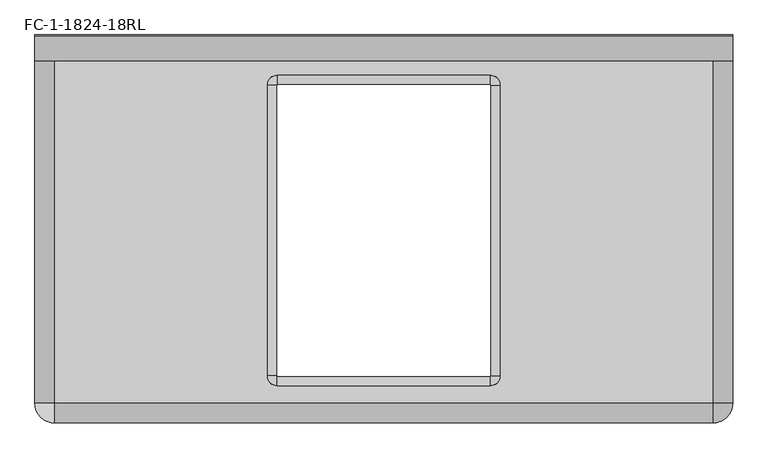
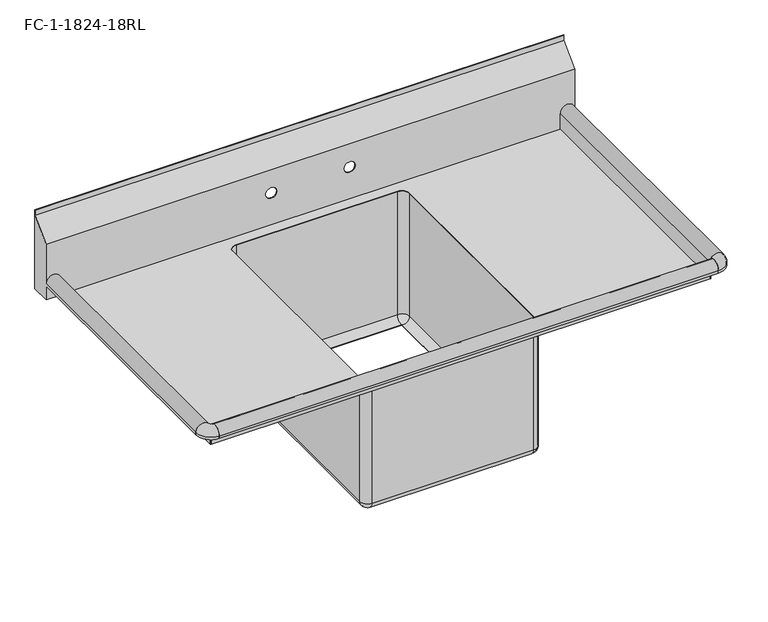
"""IFC4 building model written with IfcOpenShell, lengths in millimetres: proxy geometry, qf_advance_fc-1$2014$FC-1-1824-18RL : FC-1-1824-18RL."""

from ifc_helpers import new_model, si_unit, point, frame, frame_2d, origin, place, context, project, spatial, polyline, circle_curve, ellipse_curve, trimmed, segment, composite_curve, outline, extrude, source, transform, mapped, element, save
from ifc_brep_helpers import plane_surface, cylinder_surface, revolved_surface, advanced_brep


def fc_1_1824_18rl_eb121c77(model_context):
    return source(origin(), model_context, "Body", "SolidModel", [
        advanced_brep(
        [(915.9680523, -98.425, 539.7540518), (895.35, -77.8069477, 539.7540518), (895.35, -77.8069477, 876.3), (915.9680523, -98.425, 876.3), (896.9063565, -98.425, 520.692356), (895.35, -96.8686435, 520.692356), (896.9063565, -98.425, 522.2798689), (895.35, -96.8686435, 522.2798689), (914.3805538, -98.425, 539.7540662), (895.35, -79.3944462, 539.7540662), (914.3805538, -98.425, 876.3), (895.35, -79.3944462, 876.3), (915.9680523, -669.925, 876.3), (915.9680523, -669.925, 539.7540518), (896.9063565, -669.925, 520.692356), (896.9063565, -669.925, 522.2798689), (914.3805538, -669.925, 539.7540662), (914.3805538, -669.925, 876.3), (895.35, -690.5430523, 539.7540518), (895.35, -690.5430523, 876.3), (895.35, -671.4813565, 520.692356), (895.35, -671.4813565, 522.2798689), (895.35, -688.9555538, 539.7540662), (895.35, -688.9555538, 876.3), (476.25, -690.5430523, 876.3), (476.25, -690.5430523, 539.7540518), (476.25, -671.4813565, 520.692356), (476.25, -671.4813565, 522.2798689), (476.25, -688.9555538, 539.7540662), (476.25, -688.9555538, 876.3), (455.6319477, -669.925, 539.7540518), (455.6319477, -669.925, 876.3), (474.6936435, -669.925, 520.692356), (474.6936435, -669.925, 522.2798689), (457.2194462, -669.925, 539.7540662), (457.2194462, -669.925, 876.3), (455.6319477, -98.425, 876.3), (455.6319477, -98.425, 539.7540518), (474.6936435, -98.425, 520.692356), (474.6936435, -98.425, 522.2798689), (457.2194462, -98.425, 539.7540662), (457.2194462, -98.425, 876.3), (476.25, -77.8069477, 539.7540518), (476.25, -77.8069477, 876.3), (476.25, -96.8686435, 520.692356), (476.25, -96.8686435, 522.2798689), (476.25, -79.3944462, 539.7540662), (476.25, -79.3944462, 876.3)],
        [
            (0, 1, circle_curve(frame((895.35, -98.425, 539.7540518), z_axis=(0.0, 0.0, 1.0), x_axis=(0.0, 1.0, 0.0)), 20.6180523)),
            (1, 2),
            (2, 3, circle_curve(frame((895.35, -98.425, 876.3), z_axis=(0.0, 0.0, -1.0), x_axis=(0.0, 1.0, 0.0)), 20.6180523)),
            (3, 0),
            (4, 5, circle_curve(frame((895.35, -98.425, 520.692356), z_axis=(0.0, 0.0, 1.0), x_axis=(0.0, 1.0, 0.0)), 1.5563565)),
            (5, 1, circle_curve(frame((895.35, -96.8686435, 539.7540518), z_axis=(1.0, 0.0, 0.0), x_axis=(0.0, 1.0, 0.0)), 19.0616958)),
            (0, 4, circle_curve(frame((896.9063565, -98.425, 539.7540518), z_axis=(0.0, 1.0, 0.0), x_axis=(1.0, 0.0, 0.0)), 19.0616958)),
            (6, 7, circle_curve(frame((895.35, -98.425, 522.2798689), z_axis=(0.0, 0.0, 1.0), x_axis=(0.0, 1.0, 0.0)), 1.5563565)),
            (7, 5),
            (4, 6),
            (8, 9, circle_curve(frame((895.35, -98.425, 539.7540662), z_axis=(0.0, 0.0, 1.0), x_axis=(0.0, 1.0, 0.0)), 19.0305538)),
            (9, 7, circle_curve(frame((895.35, -96.8686435, 539.7540662), z_axis=(-1.0, 0.0, 0.0), x_axis=(0.0, 1.0, 0.0)), 17.4741973)),
            (6, 8, circle_curve(frame((896.9063565, -98.425, 539.7540662), z_axis=(0.0, -1.0, 0.0), x_axis=(1.0, 0.0, 0.0)), 17.4741973)),
            (10, 11, circle_curve(frame((895.35, -98.425, 876.3), z_axis=(0.0, 0.0, 1.0), x_axis=(0.0, 1.0, 0.0)), 19.0305538)),
            (11, 9),
            (8, 10),
            (3, 12),
            (12, 13),
            (13, 0),
            (13, 14, circle_curve(frame((896.9063565, -669.925, 539.7540518), z_axis=(0.0, 1.0, 0.0), x_axis=(1.0, 0.0, 0.0)), 19.0616958)),
            (14, 4),
            (14, 15),
            (15, 6),
            (15, 16, circle_curve(frame((896.9063565, -669.925, 539.7540662), z_axis=(0.0, -1.0, 0.0), x_axis=(1.0, 0.0, 0.0)), 17.4741973)),
            (16, 8),
            (16, 17),
            (17, 10),
            (18, 13, circle_curve(frame((895.35, -669.925, 539.7540518), z_axis=(0.0, 0.0, 1.0), x_axis=(1.0, 0.0, 0.0)), 20.6180523)),
            (12, 19, circle_curve(frame((895.35, -669.925, 876.3), z_axis=(0.0, 0.0, -1.0), x_axis=(1.0, 0.0, 0.0)), 20.6180523)),
            (19, 18),
            (20, 14, circle_curve(frame((895.35, -669.925, 520.692356), z_axis=(0.0, 0.0, 1.0), x_axis=(1.0, 0.0, 0.0)), 1.5563565)),
            (18, 20, circle_curve(frame((895.35, -671.4813565, 539.7540518), z_axis=(1.0, 0.0, 0.0), x_axis=(0.0, -1.0, 0.0)), 19.0616958)),
            (21, 15, circle_curve(frame((895.35, -669.925, 522.2798689), z_axis=(0.0, 0.0, 1.0), x_axis=(1.0, 0.0, 0.0)), 1.5563565)),
            (20, 21),
            (22, 16, circle_curve(frame((895.35, -669.925, 539.7540662), z_axis=(0.0, 0.0, 1.0), x_axis=(1.0, 0.0, 0.0)), 19.0305538)),
            (21, 22, circle_curve(frame((895.35, -671.4813565, 539.7540662), z_axis=(-1.0, 0.0, 0.0), x_axis=(0.0, -1.0, 0.0)), 17.4741973)),
            (23, 17, circle_curve(frame((895.35, -669.925, 876.3), z_axis=(0.0, 0.0, 1.0), x_axis=(1.0, 0.0, 0.0)), 19.0305538)),
            (22, 23),
            (19, 24),
            (24, 25),
            (25, 18),
            (25, 26, circle_curve(frame((476.25, -671.4813565, 539.7540518), z_axis=(1.0, 0.0, 0.0), x_axis=(0.0, -1.0, 0.0)), 19.0616958)),
            (26, 20),
            (26, 27),
            (27, 21),
            (27, 28, circle_curve(frame((476.25, -671.4813565, 539.7540662), z_axis=(-1.0, 0.0, 0.0), x_axis=(0.0, -1.0, 0.0)), 17.4741973)),
            (28, 22),
            (28, 29),
            (29, 23),
            (30, 25, circle_curve(frame((476.25, -669.925, 539.7540518), z_axis=(0.0, 0.0, 1.0), x_axis=(0.0, -1.0, 0.0)), 20.6180523)),
            (24, 31, circle_curve(frame((476.25, -669.925, 876.3), z_axis=(0.0, 0.0, -1.0), x_axis=(0.0, -1.0, 0.0)), 20.6180523)),
            (31, 30),
            (32, 26, circle_curve(frame((476.25, -669.925, 520.692356), z_axis=(0.0, 0.0, 1.0), x_axis=(0.0, -1.0, 0.0)), 1.5563565)),
            (30, 32, circle_curve(frame((474.6936435, -669.925, 539.7540518), z_axis=(0.0, -1.0, 0.0), x_axis=(-1.0, 0.0, 0.0)), 19.0616958)),
            (33, 27, circle_curve(frame((476.25, -669.925, 522.2798689), z_axis=(0.0, 0.0, 1.0), x_axis=(0.0, -1.0, 0.0)), 1.5563565)),
            (32, 33),
            (34, 28, circle_curve(frame((476.25, -669.925, 539.7540662), z_axis=(0.0, 0.0, 1.0), x_axis=(0.0, -1.0, 0.0)), 19.0305538)),
            (33, 34, circle_curve(frame((474.6936435, -669.925, 539.7540662), z_axis=(0.0, 1.0, 0.0), x_axis=(-1.0, 0.0, 0.0)), 17.4741973)),
            (35, 29, circle_curve(frame((476.25, -669.925, 876.3), z_axis=(0.0, 0.0, 1.0), x_axis=(0.0, -1.0, 0.0)), 19.0305538)),
            (34, 35),
            (31, 36),
            (36, 37),
            (37, 30),
            (37, 38, circle_curve(frame((474.6936435, -98.425, 539.7540518), z_axis=(0.0, -1.0, 0.0), x_axis=(-1.0, 0.0, 0.0)), 19.0616958)),
            (38, 32),
            (38, 39),
            (39, 33),
            (39, 40, circle_curve(frame((474.6936435, -98.425, 539.7540662), z_axis=(0.0, 1.0, 0.0), x_axis=(-1.0, 0.0, 0.0)), 17.4741973)),
            (40, 34),
            (40, 41),
            (41, 35),
            (42, 37, circle_curve(frame((476.25, -98.425, 539.7540518), z_axis=(0.0, 0.0, 1.0), x_axis=(-1.0, 0.0, 0.0)), 20.6180523)),
            (36, 43, circle_curve(frame((476.25, -98.425, 876.3), z_axis=(0.0, 0.0, -1.0), x_axis=(-1.0, 0.0, 0.0)), 20.6180523)),
            (43, 42),
            (44, 38, circle_curve(frame((476.25, -98.425, 520.692356), z_axis=(0.0, 0.0, 1.0), x_axis=(-1.0, 0.0, 0.0)), 1.5563565)),
            (42, 44, circle_curve(frame((476.25, -96.8686435, 539.7540518), z_axis=(-1.0, 0.0, 0.0), x_axis=(0.0, 1.0, 0.0)), 19.0616958)),
            (45, 39, circle_curve(frame((476.25, -98.425, 522.2798689), z_axis=(0.0, 0.0, 1.0), x_axis=(-1.0, 0.0, 0.0)), 1.5563565)),
            (44, 45),
            (46, 40, circle_curve(frame((476.25, -98.425, 539.7540662), z_axis=(0.0, 0.0, 1.0), x_axis=(-1.0, 0.0, 0.0)), 19.0305538)),
            (45, 46, circle_curve(frame((476.25, -96.8686435, 539.7540662), z_axis=(1.0, 0.0, 0.0), x_axis=(0.0, 1.0, 0.0)), 17.4741973)),
            (47, 41, circle_curve(frame((476.25, -98.425, 876.3), z_axis=(0.0, 0.0, 1.0), x_axis=(-1.0, 0.0, 0.0)), 19.0305538)),
            (46, 47),
            (43, 2),
            (1, 42),
            (5, 44),
            (7, 45),
            (9, 46),
            (11, 47),
        ],
        [
            cylinder_surface(frame((895.35, -98.425, 0.0), z_axis=(0.0, 0.0, -1.0), x_axis=(0.0, 1.0, 0.0)), 20.6180523),
            revolved_surface(trimmed(ellipse_curve(frame((895.35, -96.8686435, 539.7540518), z_axis=(-1.0, 0.0, 0.0), x_axis=(0.0, 1.0, 0.0)), 19.0616958, 19.0616958), [point((895.35, -77.8069477, 539.7540518))], [point((895.35, -96.8686435, 520.692356))], True, "CARTESIAN"), (895.35, -98.425, 0.0), (0.0, 0.0, -1.0)),
            revolved_surface(polyline([(895.35, -96.86864349999999, 520.692356), (895.35, -96.86864349999999, 522.2798689)]), (895.35, -98.425, 0.0), (0.0, 0.0, -1.0)),
            revolved_surface(trimmed(ellipse_curve(frame((895.35, -96.8686435, 539.7540662), z_axis=(1.0, 0.0, 0.0), x_axis=(0.0, 1.0, 0.0)), 17.4741973, 17.4741973), [point((895.35, -96.8686435, 522.2798689))], [point((895.35, -79.3944462, 539.7540662))], True, "CARTESIAN"), (895.35, -98.425, 0.0), (0.0, 0.0, -1.0)),
            revolved_surface(polyline([(895.35, -79.3944462, 539.7540662), (895.35, -79.3944462, 876.3)]), (895.35, -98.425, 0.0), (0.0, 0.0, -1.0)),
            plane_surface(frame((915.9680523, -98.425, 876.3), z_axis=(1.0, 0.0, 0.0), x_axis=(0.0, -1.0, 0.0))),
            cylinder_surface(frame((896.9063565, -98.425, 539.7540518), z_axis=(0.0, 1.0, 0.0), x_axis=(1.0, 0.0, 0.0)), 19.0616958),
            plane_surface(frame((896.9063565, -98.425, 520.692356), z_axis=(-1.0, 0.0, 0.0), x_axis=(0.0, -1.0, 0.0))),
            revolved_surface(polyline([(914.3805538, -669.925, 539.7540662), (914.3805538, -98.425, 539.7540662)]), (896.9063565, -98.425, 539.7540662), (0.0, -1.0, 0.0)),
            plane_surface(frame((914.3805538, -98.425, 539.7540662), z_axis=(-1.0, 0.0, 0.0), x_axis=(0.0, -1.0, 0.0))),
            cylinder_surface(frame((895.35, -669.925, 0.0), z_axis=(0.0, 0.0, -1.0), x_axis=(1.0, 0.0, 0.0)), 20.6180523),
            revolved_surface(trimmed(ellipse_curve(frame((896.9063565, -669.925, 539.7540518), z_axis=(0.0, 1.0, 0.0), x_axis=(1.0, 0.0, 0.0)), 19.0616958, 19.0616958), [point((915.9680523, -669.925, 539.7540518))], [point((896.9063565, -669.925, 520.692356))], True, "CARTESIAN"), (895.35, -669.925, 0.0), (0.0, 0.0, -1.0)),
            revolved_surface(polyline([(896.9063565, -669.925, 520.692356), (896.9063565, -669.925, 522.2798689)]), (895.35, -669.925, 0.0), (0.0, 0.0, -1.0)),
            revolved_surface(trimmed(ellipse_curve(frame((896.9063565, -669.925, 539.7540662), z_axis=(0.0, -1.0, 0.0), x_axis=(1.0, 0.0, 0.0)), 17.4741973, 17.4741973), [point((896.9063565, -669.925, 522.2798689))], [point((914.3805538, -669.925, 539.7540662))], True, "CARTESIAN"), (895.35, -669.925, 0.0), (0.0, 0.0, -1.0)),
            revolved_surface(polyline([(914.3805538, -669.925, 539.7540662), (914.3805538, -669.925, 876.3)]), (895.35, -669.925, 0.0), (0.0, 0.0, -1.0)),
            plane_surface(frame((895.35, -690.5430523, 876.3), z_axis=(0.0, -1.0, 0.0), x_axis=(-1.0, 0.0, 0.0))),
            cylinder_surface(frame((895.35, -671.4813565, 539.7540518), z_axis=(1.0, 0.0, 0.0), x_axis=(0.0, -1.0, 0.0)), 19.0616958),
            plane_surface(frame((895.35, -671.4813565, 520.692356), z_axis=(0.0, 1.0, 0.0), x_axis=(-1.0, 0.0, 0.0))),
            revolved_surface(polyline([(476.25, -688.9555538, 539.7540662), (895.35, -688.9555538, 539.7540662)]), (895.35, -671.4813565, 539.7540662), (-1.0, 0.0, 0.0)),
            plane_surface(frame((895.35, -688.9555538, 539.7540662), z_axis=(0.0, 1.0, 0.0), x_axis=(-1.0, 0.0, 0.0))),
            cylinder_surface(frame((476.25, -669.925, 0.0), z_axis=(0.0, 0.0, -1.0), x_axis=(0.0, -1.0, 0.0)), 20.6180523),
            revolved_surface(trimmed(ellipse_curve(frame((476.25, -671.4813565, 539.7540518), z_axis=(1.0, 0.0, 0.0), x_axis=(0.0, -1.0, 0.0)), 19.0616958, 19.0616958), [point((476.25, -690.5430523, 539.7540518))], [point((476.25, -671.4813565, 520.692356))], True, "CARTESIAN"), (476.25, -669.925, 0.0), (0.0, 0.0, -1.0)),
            revolved_surface(polyline([(476.25, -671.4813565, 520.692356), (476.25, -671.4813565, 522.2798689)]), (476.25, -669.925, 0.0), (0.0, 0.0, -1.0)),
            revolved_surface(trimmed(ellipse_curve(frame((476.25, -671.4813565, 539.7540662), z_axis=(-1.0, 0.0, 0.0), x_axis=(0.0, -1.0, 0.0)), 17.4741973, 17.4741973), [point((476.25, -671.4813565, 522.2798689))], [point((476.25, -688.9555538, 539.7540662))], True, "CARTESIAN"), (476.25, -669.925, 0.0), (0.0, 0.0, -1.0)),
            revolved_surface(polyline([(476.25, -688.9555538, 539.7540662), (476.25, -688.9555538, 876.3)]), (476.25, -669.925, 0.0), (0.0, 0.0, -1.0)),
            plane_surface(frame((455.6319477, -669.925, 876.3), z_axis=(-1.0, 0.0, 0.0), x_axis=(0.0, 1.0, 0.0))),
            cylinder_surface(frame((474.6936435, -669.925, 539.7540518), z_axis=(0.0, -1.0, 0.0), x_axis=(-1.0, 0.0, 0.0)), 19.0616958),
            plane_surface(frame((474.6936435, -669.925, 520.692356), z_axis=(1.0, 0.0, 0.0), x_axis=(0.0, 1.0, 0.0))),
            revolved_surface(polyline([(457.2194462, -98.42499999999995, 539.7540662), (457.2194462, -669.925, 539.7540662)]), (474.6936435, -669.925, 539.7540662), (0.0, 1.0, 0.0)),
            plane_surface(frame((457.2194462, -669.925, 539.7540662), z_axis=(1.0, 0.0, 0.0), x_axis=(0.0, 1.0, 0.0))),
            cylinder_surface(frame((476.25, -98.425, 0.0), z_axis=(0.0, 0.0, -1.0), x_axis=(-1.0, 0.0, 0.0)), 20.6180523),
            revolved_surface(trimmed(ellipse_curve(frame((474.6936435, -98.425, 539.7540518), z_axis=(0.0, -1.0, 0.0), x_axis=(-1.0, 0.0, 0.0)), 19.0616958, 19.0616958), [point((455.6319477, -98.425, 539.7540518))], [point((474.6936435, -98.425, 520.692356))], True, "CARTESIAN"), (476.25, -98.425, 0.0), (0.0, 0.0, -1.0)),
            revolved_surface(polyline([(474.6936435, -98.425, 520.692356), (474.6936435, -98.425, 522.2798689)]), (476.25, -98.425, 0.0), (0.0, 0.0, -1.0)),
            revolved_surface(trimmed(ellipse_curve(frame((474.6936435, -98.425, 539.7540662), z_axis=(0.0, 1.0, 0.0), x_axis=(-1.0, 0.0, 0.0)), 17.4741973, 17.4741973), [point((474.6936435, -98.425, 522.2798689))], [point((457.2194462, -98.425, 539.7540662))], True, "CARTESIAN"), (476.25, -98.425, 0.0), (0.0, 0.0, -1.0)),
            revolved_surface(polyline([(457.2194462, -98.425, 539.7540662), (457.2194462, -98.425, 876.3)]), (476.25, -98.425, 0.0), (0.0, 0.0, -1.0)),
            plane_surface(frame((476.25, -77.8069477, 876.3), z_axis=(0.0, 1.0, 0.0), x_axis=(1.0, 0.0, 0.0))),
            cylinder_surface(frame((476.25, -96.8686435, 539.7540518), z_axis=(-1.0, 0.0, 0.0), x_axis=(0.0, 1.0, 0.0)), 19.0616958),
            plane_surface(frame((476.25, -96.8686435, 520.692356), z_axis=(0.0, -1.0, 0.0), x_axis=(1.0, 0.0, 0.0))),
            revolved_surface(polyline([(895.35, -79.3944462, 539.7540662), (476.25, -79.3944462, 539.7540662)]), (476.25, -96.8686435, 539.7540662), (1.0, 0.0, 0.0)),
            plane_surface(frame((476.25, -79.3944462, 539.7540662), z_axis=(0.0, -1.0, 0.0), x_axis=(1.0, 0.0, 0.0))),
            plane_surface(frame((476.25, -79.3944462, 876.3), z_axis=(0.0, 0.0, 1.0), x_axis=(1.0, 0.0, 0.0))),
        ],
        [
            (0, [[1, 2, 3, 4]]),
            (1, [[5, 6, -1, 7]]),
            (2, [[8, 9, -5, 10]]),
            (3, [[11, 12, -8, 13]]),
            (4, [[14, 15, -11, 16]]),
            (5, [[-4, 17, 18, 19]]),
            (6, [[-7, -19, 20, 21]]),
            (7, [[-10, -21, 22, 23]]),
            (8, [[-13, -23, 24, 25]]),
            (9, [[-16, -25, 26, 27]]),
            (10, [[28, -18, 29, 30]]),
            (11, [[31, -20, -28, 32]]),
            (12, [[33, -22, -31, 34]]),
            (13, [[35, -24, -33, 36]]),
            (14, [[37, -26, -35, 38]]),
            (15, [[-30, 39, 40, 41]]),
            (16, [[-32, -41, 42, 43]]),
            (17, [[-34, -43, 44, 45]]),
            (18, [[-36, -45, 46, 47]]),
            (19, [[-38, -47, 48, 49]]),
            (20, [[50, -40, 51, 52]]),
            (21, [[53, -42, -50, 54]]),
            (22, [[55, -44, -53, 56]]),
            (23, [[57, -46, -55, 58]]),
            (24, [[59, -48, -57, 60]]),
            (25, [[-52, 61, 62, 63]]),
            (26, [[-54, -63, 64, 65]]),
            (27, [[-56, -65, 66, 67]]),
            (28, [[-58, -67, 68, 69]]),
            (29, [[-60, -69, 70, 71]]),
            (30, [[72, -62, 73, 74]]),
            (31, [[75, -64, -72, 76]]),
            (32, [[77, -66, -75, 78]]),
            (33, [[79, -68, -77, 80]]),
            (34, [[81, -70, -79, 82]]),
            (35, [[-74, 83, -2, 84]]),
            (36, [[-76, -84, -6, 85]]),
            (37, [[-78, -85, -9, 86]]),
            (38, [[-80, -86, -12, 87]]),
            (39, [[-82, -87, -15, 88]]),
            (40, [[-83, -73, -61, -51, -39, -29, -17, -3], [-71, -81, -88, -14, -27, -37, -49, -59]]),
        ],
    ),
        extrude(outline(polyline([(38.1, -723.9), (38.1, -50.8), (1333.5, -50.8), (1333.5, -723.9), (38.1, -723.9)]), holes=[composite_curve([segment(trimmed(circle_curve(frame_2d((895.35, -98.425)), 19.05), [point((914.4, -98.425))], [point((895.35, -79.375))], True, "CARTESIAN"), True, "CONTINUOUS"), segment(polyline([(895.35, -79.375), (476.25, -79.375)]), True, "CONTINUOUS"), segment(trimmed(circle_curve(frame_2d((476.25, -98.425)), 19.05), [point((476.25, -79.375))], [point((457.2, -98.425))], True, "CARTESIAN"), True, "CONTINUOUS"), segment(polyline([(457.2, -98.425), (457.2, -669.925)]), True, "CONTINUOUS"), segment(trimmed(circle_curve(frame_2d((476.25, -669.925)), 19.05), [point((457.2, -669.925))], [point((476.25, -688.975))], True, "CARTESIAN"), True, "CONTINUOUS"), segment(polyline([(476.25, -688.975), (895.35, -688.975)]), True, "CONTINUOUS"), segment(trimmed(circle_curve(frame_2d((895.35, -669.925)), 19.05), [point((895.35, -688.975))], [point((914.4, -669.925))], True, "CARTESIAN"), True, "CONTINUOUS"), segment(polyline([(914.4, -669.925), (914.4, -98.425)]), True, "CONTINUOUS")], self_intersect=False)]), frame((0.0, 0.0, 876.3), z_axis=(0.0, 0.0, 1.0), x_axis=(1.0, 0.0, 0.0)), (0.0, 0.0, 1.0), 1.5875),
        advanced_brep(
        [(38.1, -725.4875, 876.3), (38.1, -723.9, 876.3), (38.1, -723.9, 920.75), (38.1, -762.0, 920.75), (38.1, -762.0, 914.4), (38.1, -760.4125, 914.4), (38.1, -760.4125, 920.75), (38.1, -725.4875, 920.75), (36.5125, -723.9, 876.3), (36.5125, -723.9, 920.75), (1.5875, -723.9, 920.75), (1.5875, -723.9, 914.4), (0.0, -723.9, 914.4), (0.0, -723.9, 920.75)],
        [
            (0, 1),
            (1, 2),
            (2, 3, circle_curve(frame((38.1, -742.95, 920.75), z_axis=(1.0, 0.0, 0.0), x_axis=(0.0, -1.0, 0.0)), 19.05)),
            (3, 4),
            (4, 5),
            (5, 6),
            (6, 7, circle_curve(frame((38.1, -742.95, 920.75), z_axis=(-1.0, 0.0, 0.0), x_axis=(0.0, -1.0, 0.0)), 17.4625)),
            (7, 0),
            (8, 9),
            (9, 10, circle_curve(frame((19.05, -723.9, 920.75), z_axis=(0.0, -1.0, 0.0), x_axis=(-1.0, 0.0, 0.0)), 17.4625)),
            (10, 11),
            (11, 12),
            (12, 13),
            (13, 2, circle_curve(frame((19.05, -723.9, 920.75), z_axis=(0.0, 1.0, 0.0), x_axis=(-1.0, 0.0, 0.0)), 19.05)),
            (1, 8),
            (8, 0, circle_curve(frame((38.1, -723.9, 876.3), z_axis=(0.0, 0.0, 1.0), x_axis=(0.0, -1.0, 0.0)), 1.5875)),
            (7, 9, circle_curve(frame((38.1, -723.9, 920.75), z_axis=(0.0, 0.0, -1.0), x_axis=(0.0, -1.0, 0.0)), 1.5875)),
            (6, 10, circle_curve(frame((38.1, -723.9, 920.75), z_axis=(0.0, 0.0, -1.0), x_axis=(0.0, -1.0, 0.0)), 36.5125)),
            (5, 11, circle_curve(frame((38.1, -723.9, 914.4), z_axis=(0.0, 0.0, -1.0), x_axis=(0.0, -1.0, 0.0)), 36.5125)),
            (4, 12, circle_curve(frame((38.1, -723.9, 914.4), z_axis=(0.0, 0.0, -1.0), x_axis=(0.0, -1.0, 0.0)), 38.1)),
            (3, 13, circle_curve(frame((38.1, -723.9, 920.75), z_axis=(0.0, 0.0, -1.0), x_axis=(0.0, -1.0, 0.0)), 38.1)),
        ],
        [
            plane_surface(frame((38.1, -723.9, 876.3), z_axis=(1.0, 0.0, 0.0), x_axis=(0.0, -1.0, 0.0))),
            plane_surface(frame((38.1, -723.9, 876.3), z_axis=(0.0, 1.0, 0.0), x_axis=(-1.0, 0.0, 0.0))),
            cylinder_surface(frame((38.1, -723.9, 876.3), z_axis=(0.0, 0.0, -1.0), x_axis=(0.0, -1.0, 0.0)), 1.5875),
            revolved_surface(trimmed(ellipse_curve(frame((38.1, -742.95, 920.75), z_axis=(-1.0, 0.0, 0.0), x_axis=(0.0, -1.0, 0.0)), 17.4625, 17.4625), [point((38.1, -760.4125, 920.75))], [point((38.1, -725.4875, 920.75))], True, "CARTESIAN"), (38.1, -723.9, 876.3), (0.0, 0.0, -1.0)),
            revolved_surface(polyline([(38.1, -760.4125, 914.4), (38.1, -760.4125, 920.75)]), (38.1, -723.9, 876.3), (0.0, 0.0, -1.0)),
            plane_surface(frame((38.1, -723.9, 914.4), z_axis=(0.0, 0.0, -1.0), x_axis=(0.0, -1.0, 0.0))),
            cylinder_surface(frame((38.1, -723.9, 876.3), z_axis=(0.0, 0.0, -1.0), x_axis=(0.0, -1.0, 0.0)), 38.1),
            revolved_surface(trimmed(ellipse_curve(frame((38.1, -742.95, 920.75), z_axis=(1.0, 0.0, 0.0), x_axis=(0.0, -1.0, 0.0)), 19.05, 19.05), [point((38.1, -723.9, 920.75))], [point((38.1, -762.0, 920.75))], True, "CARTESIAN"), (38.1, -723.9, 876.3), (0.0, 0.0, -1.0)),
            plane_surface(frame((38.1, -723.9, 876.3), z_axis=(0.0, 0.0, -1.0), x_axis=(0.0, -1.0, 0.0))),
        ],
        [
            (0, [[1, 2, 3, 4, 5, 6, 7, 8]]),
            (1, [[9, 10, 11, 12, 13, 14, -2, 15]]),
            (2, [[16, -8, 17, -9]]),
            (3, [[-17, -7, 18, -10]]),
            (4, [[-18, -6, 19, -11]]),
            (5, [[-19, -5, 20, -12]]),
            (6, [[-20, -4, 21, -13]]),
            (7, [[-21, -3, -14]]),
            (8, [[-1, -16, -15]]),
        ],
    ),
        advanced_brep(
        [(1333.5, -725.4875, 876.3), (1333.5, -725.4875, 920.75), (1333.5, -760.4125, 920.75), (1333.5, -760.4125, 914.4), (1333.5, -762.0, 914.4), (1333.5, -762.0, 920.75), (1333.5, -723.9, 920.75), (1333.5, -723.9, 876.3), (1335.0875, -723.9, 876.3), (1371.6, -723.9, 920.75), (1371.6, -723.9, 914.4), (1370.0125, -723.9, 914.4), (1370.0125, -723.9, 920.75), (1335.0875, -723.9, 920.75)],
        [
            (0, 1),
            (1, 2, circle_curve(frame((1333.5, -742.95, 920.75), z_axis=(1.0, 0.0, 0.0), x_axis=(0.0, -1.0, 0.0)), 17.4625)),
            (2, 3),
            (3, 4),
            (4, 5),
            (5, 6, circle_curve(frame((1333.5, -742.95, 920.75), z_axis=(-1.0, 0.0, 0.0), x_axis=(0.0, -1.0, 0.0)), 19.05)),
            (6, 7),
            (7, 0),
            (8, 7),
            (6, 9, circle_curve(frame((1352.55, -723.9, 920.75), z_axis=(0.0, 1.0, 0.0), x_axis=(1.0, 0.0, 0.0)), 19.05)),
            (9, 10),
            (10, 11),
            (11, 12),
            (12, 13, circle_curve(frame((1352.55, -723.9, 920.75), z_axis=(0.0, -1.0, 0.0), x_axis=(1.0, 0.0, 0.0)), 17.4625)),
            (13, 8),
            (13, 1, circle_curve(frame((1333.5, -723.9, 920.75), z_axis=(0.0, 0.0, -1.0), x_axis=(0.0, -1.0, 0.0)), 1.5875)),
            (0, 8, circle_curve(frame((1333.5, -723.9, 876.3), z_axis=(0.0, 0.0, 1.0), x_axis=(0.0, -1.0, 0.0)), 1.5875)),
            (12, 2, circle_curve(frame((1333.5, -723.9, 920.75), z_axis=(0.0, 0.0, -1.0), x_axis=(0.0, -1.0, 0.0)), 36.5125)),
            (11, 3, circle_curve(frame((1333.5, -723.9, 914.4), z_axis=(0.0, 0.0, -1.0), x_axis=(0.0, -1.0, 0.0)), 36.5125)),
            (10, 4, circle_curve(frame((1333.5, -723.9, 914.4), z_axis=(0.0, 0.0, -1.0), x_axis=(0.0, -1.0, 0.0)), 38.1)),
            (9, 5, circle_curve(frame((1333.5, -723.9, 920.75), z_axis=(0.0, 0.0, -1.0), x_axis=(0.0, -1.0, 0.0)), 38.1)),
        ],
        [
            plane_surface(frame((1333.5, -723.9, 876.3), z_axis=(-1.0, 0.0, 0.0), x_axis=(0.0, -1.0, 0.0))),
            plane_surface(frame((1333.5, -723.9, 876.3), z_axis=(0.0, 1.0, 0.0), x_axis=(1.0, 0.0, 0.0))),
            cylinder_surface(frame((1333.5, -723.9, 876.3), z_axis=(0.0, 0.0, 1.0), x_axis=(0.0, -1.0, 0.0)), 1.5875),
            revolved_surface(trimmed(ellipse_curve(frame((1333.5, -742.95, 920.75), z_axis=(1.0, 0.0, 0.0), x_axis=(0.0, -1.0, 0.0)), 17.4625, 17.4625), [point((1333.5, -725.4875, 920.75))], [point((1333.5, -760.4125, 920.75))], True, "CARTESIAN"), (1333.5, -723.9, 876.3), (0.0, 0.0, 1.0)),
            revolved_surface(polyline([(1333.5, -760.4125, 920.75), (1333.5, -760.4125, 914.4)]), (1333.5, -723.9, 876.3), (0.0, 0.0, 1.0)),
            plane_surface(frame((1333.5, -723.9, 914.4), z_axis=(0.0, 0.0, -1.0), x_axis=(0.0, -1.0, 0.0))),
            cylinder_surface(frame((1333.5, -723.9, 876.3), z_axis=(0.0, 0.0, 1.0), x_axis=(0.0, -1.0, 0.0)), 38.1),
            revolved_surface(trimmed(ellipse_curve(frame((1333.5, -742.95, 920.75), z_axis=(-1.0, 0.0, 0.0), x_axis=(0.0, -1.0, 0.0)), 19.05, 19.05), [point((1333.5, -762.0, 920.75))], [point((1333.5, -723.9, 920.75))], True, "CARTESIAN"), (1333.5, -723.9, 876.3), (0.0, 0.0, 1.0)),
            plane_surface(frame((1333.5, -723.9, 876.3), z_axis=(0.0, 0.0, -1.0), x_axis=(0.0, -1.0, 0.0))),
        ],
        [
            (0, [[1, 2, 3, 4, 5, 6, 7, 8]]),
            (1, [[9, -7, 10, 11, 12, 13, 14, 15]]),
            (2, [[16, -1, 17, -15]]),
            (3, [[18, -2, -16, -14]]),
            (4, [[19, -3, -18, -13]]),
            (5, [[20, -4, -19, -12]]),
            (6, [[21, -5, -20, -11]]),
            (7, [[-6, -21, -10]]),
            (8, [[-17, -8, -9]]),
        ],
    ),
        extrude(outline(composite_curve([segment(trimmed(circle_curve(frame_2d((-742.95, 920.75)), 19.05), [point((-762.0, 920.75))], [point((-723.9, 920.75))], False, "CARTESIAN"), True, "CONTINUOUS"), segment(polyline([(-723.9, 920.75), (-723.9, 876.3), (-725.4875, 876.3), (-725.4875, 920.75)]), True, "CONTINUOUS"), segment(trimmed(circle_curve(frame_2d((-742.95, 920.75)), 17.4625), [point((-725.4875, 920.75))], [point((-760.4125, 920.75))], True, "CARTESIAN"), True, "CONTINUOUS"), segment(polyline([(-760.4125, 920.75), (-760.4125, 914.4), (-762.0, 914.4), (-762.0, 920.75)]), True, "CONTINUOUS")], self_intersect=False)), frame((38.1, 0.0, 0.0), z_axis=(1.0, 0.0, 0.0), x_axis=(0.0, 1.0, 0.0)), (0.0, 0.0, 1.0), 1295.4),
        advanced_brep(
        [(1371.6, 0.0, 1079.5), (1371.6, 0.0, 1092.2), (1371.6, -1.5875, 1092.2), (1371.6, -1.5875, 1077.9125), (1371.6, -50.8, 1028.7), (1371.6, -50.8, 920.75), (1371.6, -723.9, 920.75), (1371.6, -723.9, 914.4), (1371.6, -50.8, 914.4), (1371.6, -50.8, 876.3), (1371.6, 0.0, 876.3), (0.0, -50.8, 1028.7), (0.0, -1.5875, 1077.9125), (0.0, -1.5875, 1092.2), (0.0, 0.0, 1092.2), (0.0, 0.0, 1079.5), (0.0, 0.0, 876.3), (0.0, -50.8, 876.3), (0.0, -50.8, 914.4), (0.0, -723.9, 914.4), (0.0, -723.9, 920.75), (0.0, -50.8, 920.75), (1370.0125, -50.8, 914.4), (1370.0125, -50.8, 920.75), (1335.0875, -50.8, 920.75), (1335.0875, -50.8, 876.3), (36.5125, -50.8, 876.3), (36.5125, -50.8, 920.75), (1.5875, -50.8, 920.75), (1.5875, -50.8, 914.4), (1.2426734, -50.8, 1028.7), (38.1, -50.8, 920.75), (38.1, -50.8, 876.3), (1333.5, -50.8, 876.3), (1333.5, -50.8, 920.75), (1370.0125, -50.8, 1028.7), (598.4875, -50.8, 965.2), (569.9125, -50.8, 965.2), (801.6875, -50.8, 965.2), (773.1125, -50.8, 965.2), (1.2426734, 0.0, 876.3), (1.2426734, -49.2125, 876.3), (1370.0125, -49.2125, 876.3), (1370.0125, 0.0, 876.3), (1335.0875, -723.9, 876.3), (1333.5, -723.9, 876.3), (38.1, -723.9, 876.3), (36.5125, -723.9, 876.3), (1.2426734, -49.2125, 1028.042436), (1370.0125, -49.2125, 1028.042436), (569.9125, -49.2125, 965.2), (598.4875, -49.2125, 965.2), (773.1125, -49.2125, 965.2), (801.6875, -49.2125, 965.2), (1.2426734, 0.0, 1077.254936), (1370.0125, 0.0, 1077.254936), (1370.0125, -1.5875, 1077.9125), (1.2426734, -1.5875, 1077.9125), (1.2426734, 0.0, 1079.5), (1370.0125, 0.0, 1079.5), (1333.5, -723.9, 920.75), (1335.0875, -723.9, 920.75), (1370.0125, -723.9, 920.75), (1370.0125, -723.9, 914.4), (1.5875, -723.9, 914.4), (1.5875, -723.9, 920.75), (36.5125, -723.9, 920.75), (38.1, -723.9, 920.75)],
        [
            (0, 1),
            (1, 2),
            (2, 3),
            (3, 4),
            (4, 5),
            (5, 6),
            (6, 7),
            (7, 8),
            (8, 9),
            (9, 10),
            (10, 0),
            (11, 12),
            (12, 13),
            (13, 14),
            (14, 15),
            (15, 16),
            (16, 17),
            (17, 18),
            (18, 19),
            (19, 20),
            (20, 21),
            (21, 11),
            (8, 22),
            (22, 23),
            (23, 24, circle_curve(frame((1352.55, -50.8, 920.75), z_axis=(0.0, -1.0, 0.0), x_axis=(1.0, 0.0, 0.0)), 17.4625)),
            (24, 25),
            (25, 9),
            (17, 26),
            (26, 27),
            (27, 28, circle_curve(frame((19.05, -50.8, 920.75), z_axis=(0.0, -1.0, 0.0), x_axis=(1.0, 0.0, 0.0)), 17.4625)),
            (28, 29),
            (29, 18),
            (30, 11),
            (21, 31, circle_curve(frame((19.05, -50.8, 920.75), z_axis=(0.0, 1.0, 0.0), x_axis=(1.0, 0.0, 0.0)), 19.05)),
            (31, 32),
            (32, 33),
            (33, 34),
            (34, 5, circle_curve(frame((1352.55, -50.8, 920.75), z_axis=(0.0, 1.0, 0.0), x_axis=(1.0, 0.0, 0.0)), 19.05)),
            (4, 35),
            (35, 30),
            (36, 37, circle_curve(frame((584.2, -50.8, 965.2), z_axis=(0.0, 1.0, 0.0), x_axis=(1.0, 0.0, 0.0)), 14.2875)),
            (37, 36, circle_curve(frame((584.2, -50.8, 965.2), z_axis=(0.0, 1.0, 0.0), x_axis=(1.0, 0.0, 0.0)), 14.2875)),
            (38, 39, circle_curve(frame((787.4, -50.8, 965.2), z_axis=(0.0, 1.0, 0.0), x_axis=(1.0, 0.0, 0.0)), 14.2875)),
            (39, 38, circle_curve(frame((787.4, -50.8, 965.2), z_axis=(0.0, 1.0, 0.0), x_axis=(1.0, 0.0, 0.0)), 14.2875)),
            (16, 40),
            (40, 41),
            (41, 42),
            (42, 43),
            (43, 10),
            (25, 44),
            (44, 45),
            (45, 33),
            (32, 46),
            (46, 47),
            (47, 26),
            (41, 48),
            (48, 49),
            (49, 42),
            (50, 51, circle_curve(frame((584.2, -49.2125, 965.2), z_axis=(0.0, -1.0, 0.0), x_axis=(1.0, 0.0, 0.0)), 14.2875)),
            (51, 50, circle_curve(frame((584.2, -49.2125, 965.2), z_axis=(0.0, -1.0, 0.0), x_axis=(1.0, 0.0, 0.0)), 14.2875)),
            (52, 53, circle_curve(frame((787.4, -49.2125, 965.2), z_axis=(0.0, -1.0, 0.0), x_axis=(1.0, 0.0, 0.0)), 14.2875)),
            (53, 52, circle_curve(frame((787.4, -49.2125, 965.2), z_axis=(0.0, -1.0, 0.0), x_axis=(1.0, 0.0, 0.0)), 14.2875)),
            (48, 54),
            (54, 55),
            (55, 49),
            (3, 56),
            (56, 57),
            (57, 12),
            (40, 54),
            (55, 43),
            (15, 58),
            (58, 59),
            (59, 0),
            (14, 1),
            (13, 2),
            (6, 60, circle_curve(frame((1352.55, -723.9, 920.75), z_axis=(0.0, -1.0, 0.0), x_axis=(1.0, 0.0, 0.0)), 19.05)),
            (60, 45),
            (44, 61),
            (61, 62, circle_curve(frame((1352.55, -723.9, 920.75), z_axis=(0.0, 1.0, 0.0), x_axis=(1.0, 0.0, 0.0)), 17.4625)),
            (62, 63),
            (63, 7),
            (63, 22),
            (62, 23),
            (61, 24),
            (60, 34),
            (19, 64),
            (64, 65),
            (65, 66, circle_curve(frame((19.05, -723.9, 920.75), z_axis=(0.0, 1.0, 0.0), x_axis=(1.0, 0.0, 0.0)), 17.4625)),
            (66, 47),
            (46, 67),
            (67, 20, circle_curve(frame((19.05, -723.9, 920.75), z_axis=(0.0, -1.0, 0.0), x_axis=(1.0, 0.0, 0.0)), 19.05)),
            (29, 64),
            (28, 65),
            (27, 66),
            (31, 67),
            (36, 51),
            (50, 37),
            (38, 53),
            (52, 39),
        ],
        [
            plane_surface(frame((1371.6, -50.8, 876.3), z_axis=(1.0, 0.0, 0.0), x_axis=(0.0, 0.0, -1.0))),
            plane_surface(frame((0.0, -50.8, 876.3), z_axis=(-1.0, 0.0, 0.0), x_axis=(0.0, 0.0, 1.0))),
            plane_surface(frame((1371.6, -50.8, 1028.7), z_axis=(0.0, -1.0, 0.0), x_axis=(-1.0, 0.0, 0.0))),
            plane_surface(frame((1371.6, -50.8, 876.3), z_axis=(0.0, 0.0, -1.0), x_axis=(-1.0, 0.0, 0.0))),
            plane_surface(frame((1371.6, -49.2125, 876.3), z_axis=(0.0, 1.0, 0.0), x_axis=(-1.0, 0.0, 0.0))),
            plane_surface(frame((1371.6, -49.2125, 1028.042436), z_axis=(0.0, 0.707106781186547, -0.707106781186548), x_axis=(-1.0, 0.0, 0.0))),
            plane_surface(frame((1371.6, -1.5875, 1077.9125), z_axis=(0.0, -0.707106781186584, 0.707106781186511), x_axis=(-1.0, 0.0, 0.0))),
            plane_surface(frame((1.2426734, 0.0, 1079.5), z_axis=(1.0, 0.0, 0.0), x_axis=(0.0, 0.0, 1.0))),
            plane_surface(frame((1370.0125, -50.8, 1028.7), z_axis=(-1.0, 0.0, 0.0), x_axis=(0.0, 0.7071067811865321, 0.7071067811865629))),
            plane_surface(frame((1371.6, 0.0, 1077.254936), z_axis=(0.0, 1.0, 0.0), x_axis=(-1.0, 0.0, 0.0))),
            plane_surface(frame((1371.6, 0.0, 1079.5), z_axis=(0.0, 1.0, 0.0), x_axis=(-1.0, 0.0, 0.0))),
            plane_surface(frame((1371.6, 0.0, 1092.2), z_axis=(0.0, 0.0, 1.0), x_axis=(-1.0, 0.0, 0.0))),
            plane_surface(frame((1371.6, -1.5875, 1092.2), z_axis=(0.0, -1.0, 0.0), x_axis=(-1.0, 0.0, 0.0))),
            plane_surface(frame((1371.6, -723.9, 0.0), z_axis=(0.0, -1.0, 0.0), x_axis=(0.0, 0.0, 1.0))),
            plane_surface(frame((1371.6, -50.8, 914.4), z_axis=(0.0, 0.0, -1.0), x_axis=(0.0, -1.0, 0.0))),
            plane_surface(frame((1370.0125, -50.8, 914.4), z_axis=(-1.0, 0.0, 0.0), x_axis=(0.0, -1.0, 0.0))),
            revolved_surface(polyline([(1370.0125, -723.9, 920.75), (1370.0125, -50.8, 920.75)]), (1352.55, -50.8, 920.75), (0.0, -1.0, 0.0)),
            plane_surface(frame((1335.0875, -50.8, 920.75), z_axis=(1.0, 0.0, 0.0), x_axis=(0.0, -1.0, 0.0))),
            plane_surface(frame((1333.5, -50.8, 876.3), z_axis=(-1.0, 0.0, 0.0), x_axis=(0.0, -1.0, 0.0))),
            cylinder_surface(frame((1352.55, -50.8, 920.75), z_axis=(0.0, 1.0, 0.0), x_axis=(1.0, 0.0, 0.0)), 19.05),
            plane_surface(frame((0.0, -723.9, 0.0), z_axis=(0.0, -1.0, 0.0), x_axis=(0.0, 0.0, 1.0))),
            plane_surface(frame((1.5875, -50.8, 914.4), z_axis=(0.0, 0.0, -1.0), x_axis=(0.0, -1.0, 0.0))),
            plane_surface(frame((1.5875, -50.8, 920.75), z_axis=(1.0, 0.0, 0.0), x_axis=(0.0, -1.0, 0.0))),
            revolved_surface(polyline([(36.5125, -723.9, 920.75), (36.5125, -50.8, 920.75)]), (19.05, -50.8, 920.75), (0.0, -1.0, 0.0)),
            plane_surface(frame((36.5125, -50.8, 876.3), z_axis=(-1.0, 0.0, 0.0), x_axis=(0.0, -1.0, 0.0))),
            plane_surface(frame((38.1, -50.8, 920.75), z_axis=(1.0, 0.0, 0.0), x_axis=(0.0, -1.0, 0.0))),
            cylinder_surface(frame((19.05, -50.8, 920.75), z_axis=(0.0, 1.0, 0.0), x_axis=(1.0, 0.0, 0.0)), 19.05),
            revolved_surface(polyline([(598.4875000000001, -50.8, 965.2), (598.4875000000001, -49.2125, 965.2)]), (584.2, -49.2125, 965.2), (0.0, -1.0, 0.0)),
            revolved_surface(polyline([(801.6875, -50.8, 965.2), (801.6875, -49.2125, 965.2)]), (787.4, 0.0, 965.2), (0.0, -1.0, 0.0)),
        ],
        [
            (0, [[1, 2, 3, 4, 5, 6, 7, 8, 9, 10, 11]]),
            (1, [[12, 13, 14, 15, 16, 17, 18, 19, 20, 21, 22]]),
            (2, [[-9, 23, 24, 25, 26, 27]]),
            (2, [[-18, 28, 29, 30, 31, 32]]),
            (2, [[33, -22, 34, 35, 36, 37, 38, -5, 39, 40], [41, 42], [43, 44]]),
            (3, [[45, 46, 47, 48, 49, -10, -27, 50, 51, 52, -36, 53, 54, 55, -28, -17]]),
            (4, [[56, 57, 58, -47], [59, 60], [61, 62]]),
            (5, [[63, 64, 65, -57]]),
            (6, [[-4, 66, 67, 68, -12, -33, -40, -39]]),
            (7, [[-46, 69, -63, -56]]),
            (8, [[-48, -58, -65, 70]]),
            (9, [[-45, -16, 71, 72, 73, -11, -49, -70, -64, -69]]),
            (10, [[-1, -73, -72, -71, -15, 74]]),
            (11, [[-2, -74, -14, 75]]),
            (12, [[-3, -75, -13, -68, -67, -66]]),
            (13, [[76, 77, -51, 78, 79, 80, 81, -7]]),
            (14, [[-81, 82, -23, -8]]),
            (15, [[-80, 83, -24, -82]]),
            (16, [[-79, 84, -25, -83]]),
            (17, [[-78, -50, -26, -84]]),
            (18, [[-77, 85, -37, -52]]),
            (19, [[-76, -6, -38, -85]]),
            (20, [[-20, 86, 87, 88, 89, -54, 90, 91]]),
            (21, [[-86, -19, -32, 92]]),
            (22, [[-87, -92, -31, 93]]),
            (23, [[-88, -93, -30, 94]]),
            (24, [[-89, -94, -29, -55]]),
            (25, [[-90, -53, -35, 95]]),
            (26, [[-91, -95, -34, -21]]),
            (27, [[96, -59, 97, -41]]),
            (27, [[-96, -42, -97, -60]]),
            (28, [[98, -61, 99, -43]]),
            (28, [[-98, -44, -99, -62]]),
        ],
    ),
    ])


if __name__ == "__main__":
    model = new_model("IFC4")
    model_context = context("Model", 3, world=origin())
    ifc_project = project(units=[si_unit("LENGTHUNIT", "METRE", prefix="MILLI")], contexts=[model_context])
    site = spatial("IfcSite", under=ifc_project)
    building = spatial("IfcBuilding", under=site)
    placement = place(None, origin())
    fc_1_1824_18rl_shape = fc_1_1824_18rl_eb121c77(model_context)
    element("IfcBuildingElementProxy", 1, Name="qf_advance_fc-1$2014$FC-1-1824-18RL : FC-1-1824-18RL", ObjectType="qf_advance_fc-1$2014$FC-1-1824-18RL : FC-1-1824-18RL", at=placement, inside=building, context=model_context, shape_type="MappedRepresentation", body=[
        mapped(fc_1_1824_18rl_shape, transform((0.0, 0.0, 0.0), x_axis=(1.0, 0.0, 0.0), y_axis=(0.0, 1.0, 0.0), z_axis=(0.0, 0.0, 1.0))),
    ])
    save(model, "model.ifc")

# Revit data of these elements
# Type "qf_advance_fc-1$2014$FC-1-1824-18RL : FC-1-1824-18RL"
#   Weight = "175 lbs."
#   URL = "www.AdvanceTabco.com"
#   Spec Sheet = "http://www.kclcutsheets.com/PDF/AD/FC_1_2Comp.pdf"
#   Model = "FC-1-1824-18RL"
#   Manufacturer = "Advance Tabco"
#   KCLRef = "KCL2C9,,000532fa-0000-0000-0000-000000000307,AD,FC-1-1824-18RL ,634763353280000000,35077c2a-8e1a-4f12-b881-d52bf8e4a175,a1de6de2-0e3a-4368-816b-f0608437979d"
#   KCL SpecSheet URL = "http://kclweb.kclcad.com/imagehandler.ashx?kdoc=fc_1_2comp&R=AD&M=FC-1-1824-18RL%20&VC=7&TID=KCLWeb&T=doc"
#   Faucet Connection = ""
#   Drain Connection = "1 1/2\" IPS"
#   Description = "16 Ga. 304 S/S Fabricated Sink, One Comp"
#   Suggested Working Height = 3' - 1"
#   Suggested Faucet Rough In = 3' - 2"
#   Right Drainboard = 1' - 6"
#   Overall Depth = 2' - 6"
#   Overall Width = 4' - 6"
#   Overall Height = 3' - 7"
#   Left Drainboard = 1' - 6"
#   Bowl Depth = 2' - 0"
#   Bowl Width = 1' - 6"
#   Water Level = 1' - 2"
#   Right And Left Cross Bracing [instance default] = yes
#   QF_Logo [instance default] = yes
#   3-1/2 Basket Drain30 = yes
#   3-1/2 Basket Drain [instance default] = no
#   QF_Finishes-Stainless Steel = QF_Finishes-Stainless Steel
#   Assembly Code = ""
# Element 1 (IfcBuildingElementProxy, "qf_advance_fc-1$2014$FC-1-1824-18RL : FC-1-1824-18RL")
#   Materials on its faces: "QF_Finishes-Stainless Steel"
# Materials
#   "QF_Finishes-Stainless Steel": class "Metal", colour RGB 127 127 127, transparency 0
